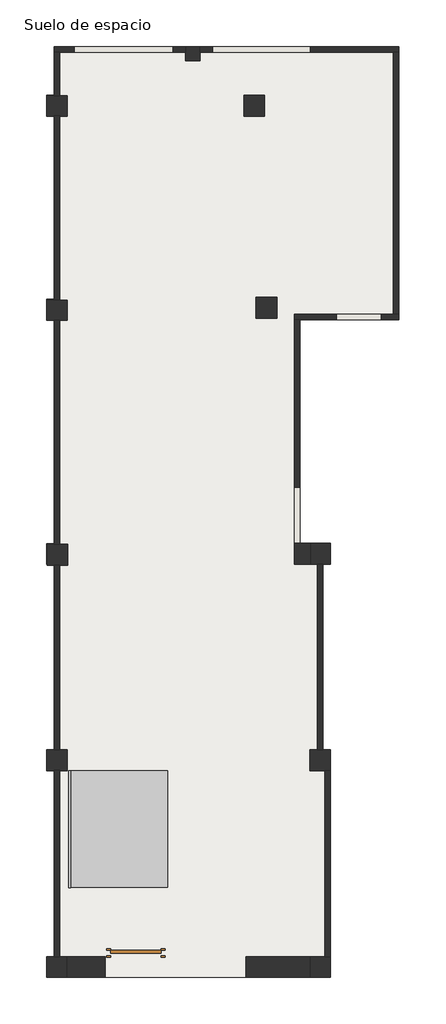
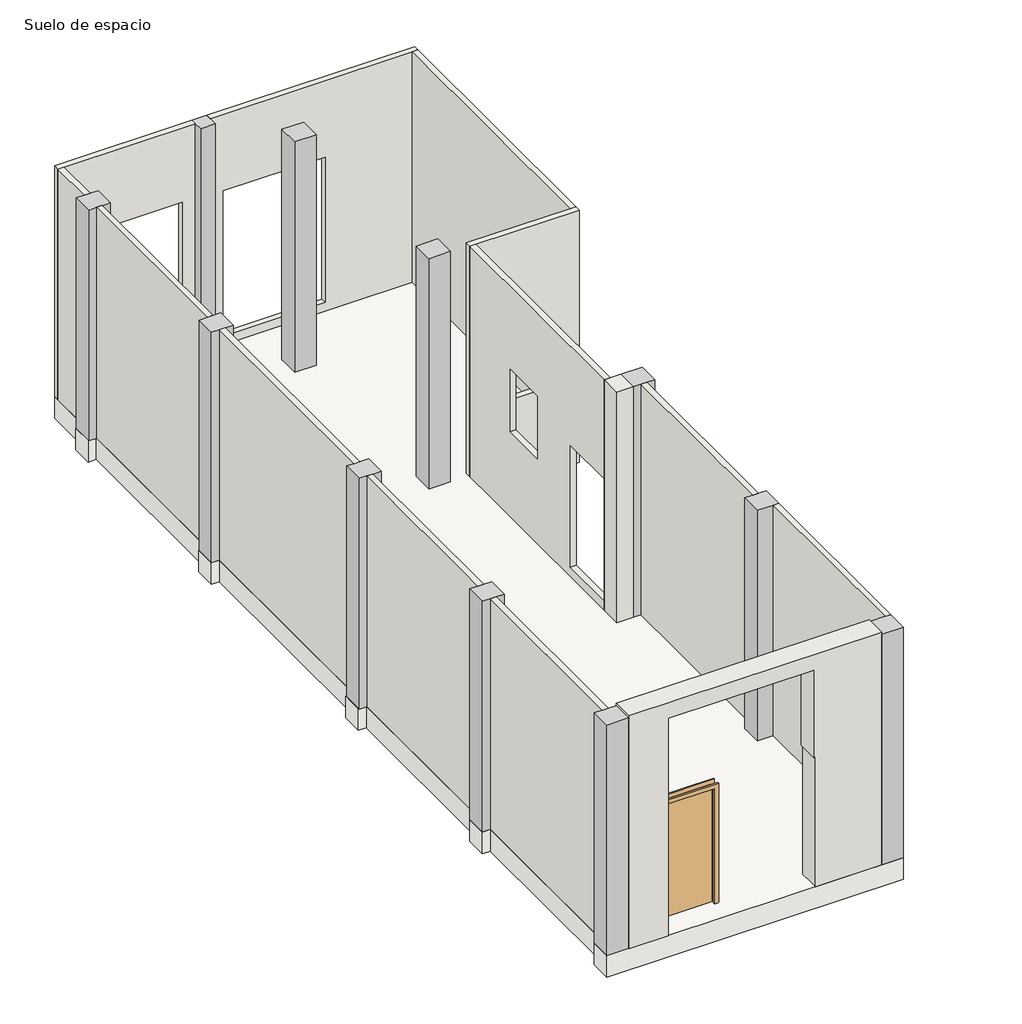
# One storey: 14 walls, 11 columns, 1 door, 1 railing, 1 ramp, 1 slab.
"""IFC4 building model written with IfcOpenShell, lengths in millimetres."""

import ifcopenshell
import ifcopenshell.guid

model = None  # the IFC model being written
_history = None  # IfcOwnerHistory: only IFC2X3 demands one
_inside = {}  # id of a spatial element -> (the spatial element, [elements in it])
_under = {}  # id of a project, library or spatial element -> (it, [spatial elements below it])
_declared = {}  # id of a project -> (the project, [libraries it declares])
_typed = {}  # id of a type object -> (the type object, [elements of that type])
_made_of = {}  # id of a material, layer set ... -> (it, [elements and type objects made of it])


def new_model(schema):
    """Start an empty IFC model of exactly this schema.

    Asked for "IFC4X3", IfcOpenShell would pick the latest addendum, in which some entities
    have other attributes; the version numbers below select the first issue.
    IFC2X3 requires an IfcOwnerHistory on every rooted entity: one is made here for all.
    """
    global model, _history
    if schema == "IFC4X3":
        model = ifcopenshell.file(schema_version=(4, 3, 0, 0))
    else:
        model = ifcopenshell.file(schema=schema)
    _inside.clear()
    _under.clear()
    _declared.clear()
    _typed.clear()
    _made_of.clear()
    _history = None
    if model.schema == "IFC2X3":
        org = make("IfcOrganization", Name="unknown")
        user = make(
            "IfcPersonAndOrganization",
            ThePerson=make("IfcPerson", FamilyName="unknown"),
            TheOrganization=org,
        )
        app = make(
            "IfcApplication",
            ApplicationDeveloper=org,
            Version="unknown",
            ApplicationFullName="unknown",
            ApplicationIdentifier="unknown",
        )
        _history = make(
            "IfcOwnerHistory",
            OwningUser=user,
            OwningApplication=app,
            ChangeAction="ADDED",
            CreationDate=0,
        )
    return model


def make(cls, **values):
    """One entity of the class cls with the attributes given. An attribute that is None is left unset."""
    return model.create_entity(
        cls, **{name: value for name, value in values.items() if value is not None}
    )


def rooted(cls, **values):
    """An entity with a GlobalId (a new one), such as an element, a storey or a relation."""
    return make(cls, GlobalId=ifcopenshell.guid.new(), OwnerHistory=_history, **values)


def si_unit(unit_type, name, prefix=None):
    """IfcSIUnit, for example si_unit("LENGTHUNIT", "METRE", prefix="MILLI")."""
    return make("IfcSIUnit", UnitType=unit_type, Prefix=prefix, Name=name)


def assignment(units):
    """IfcUnitAssignment: the units of a project."""
    return None if units is None else make("IfcUnitAssignment", Units=units)


def point(xyz):
    """IfcCartesianPoint."""
    return None if xyz is None else make("IfcCartesianPoint", Coordinates=xyz)


def direction(xyz):
    """IfcDirection."""
    return None if xyz is None else make("IfcDirection", DirectionRatios=xyz)


def frame(location, z_axis=None, x_axis=None):
    """IfcAxis2Placement3D, a coordinate frame: its origin and axes. An axis left out is left unset."""
    return make(
        "IfcAxis2Placement3D",
        Location=point(location),
        Axis=direction(z_axis),
        RefDirection=direction(x_axis),
    )


def origin():
    """The frame at (0, 0, 0) with its axes left unset."""
    return frame((0.0, 0.0, 0.0))


def origin_with_axes():
    """The frame at (0, 0, 0) with the z axis (0, 0, 1) and the x axis (1, 0, 0) written out."""
    return frame((0.0, 0.0, 0.0), z_axis=(0.0, 0.0, 1.0), x_axis=(1.0, 0.0, 0.0))


def place(relative_to, where):
    """IfcLocalPlacement: puts the frame where relative to a parent placement (None: the world)."""
    return make(
        "IfcLocalPlacement", PlacementRelTo=relative_to, RelativePlacement=where
    )


def context(
    kind, dimensions, precision=None, world=None, true_north=None, identifier=None
):
    """IfcGeometricRepresentationContext, for example the 3D "Model" context."""
    return make(
        "IfcGeometricRepresentationContext",
        ContextIdentifier=identifier,
        ContextType=kind,
        CoordinateSpaceDimension=dimensions,
        Precision=precision,
        WorldCoordinateSystem=world,
        TrueNorth=true_north,
    )


def project(units=None, contexts=None):
    """IfcProject with its units and contexts."""
    return rooted(
        "IfcProject",
        Name="project",
        RepresentationContexts=contexts,
        UnitsInContext=assignment(units),
    )


def spatial(cls, under=None, at=None, **own):
    """A site, building, storey or space (cls), placed at a placement, below another one or the project."""
    s = rooted(cls, ObjectPlacement=at, **own)
    if under is not None:
        _under.setdefault(under.id(), (under, []))[1].append(s)
    return s


def polyline(points):
    """IfcPolyline through the points."""
    return make("IfcPolyline", Points=[point(p) for p in points])


def ellipse_curve(where, semi_axis1, semi_axis2):
    """IfcEllipse in the frame where."""
    return make(
        "IfcEllipse", Position=where, SemiAxis1=semi_axis1, SemiAxis2=semi_axis2
    )


def outline(outer, holes=None, kind="AREA"):
    """IfcArbitraryClosedProfileDef: a profile drawn as a closed curve; with holes, ...WithVoids."""
    if holes is None:
        return make("IfcArbitraryClosedProfileDef", ProfileType=kind, OuterCurve=outer)
    return make(
        "IfcArbitraryProfileDefWithVoids",
        ProfileType=kind,
        OuterCurve=outer,
        InnerCurves=holes,
    )


def extrude(swept, where, along, depth):
    """IfcExtrudedAreaSolid: the profile swept, set in the frame where, extruded along a direction by depth."""
    return make(
        "IfcExtrudedAreaSolid",
        SweptArea=swept,
        Position=where,
        ExtrudedDirection=direction(along),
        Depth=depth,
    )


def faces_of(points, faces, orient=None, outer=None):
    """IfcFace entities. A face is a list of loops; a loop is a list of indices into points, from 0.

    orient and outer hold one flag for each loop. By default every Orientation is true, the
    first loop of a face is its IfcFaceOuterBound and the others are IfcFaceBound.
    """
    made = []
    for i, loops in enumerate(faces):
        bounds = []
        for j, loop in enumerate(loops):
            is_outer = j == 0 if outer is None else outer[i][j]
            bounds.append(
                make(
                    "IfcFaceOuterBound" if is_outer else "IfcFaceBound",
                    Bound=make("IfcPolyLoop", Polygon=[points[k] for k in loop]),
                    Orientation=True if orient is None else orient[i][j],
                )
            )
        made.append(make("IfcFace", Bounds=bounds))
    return made


def faceted_brep(points, faces, orient=None, outer=None, voids=None):
    """IfcFacetedBrep: a solid bounded by flat faces; with voids (closed shells), ...WithVoids."""
    shared = [point(p) for p in points]
    hull = make("IfcClosedShell", CfsFaces=faces_of(shared, faces, orient, outer))
    if voids is None:
        return make("IfcFacetedBrep", Outer=hull)
    return make(
        "IfcFacetedBrepWithVoids",
        Outer=hull,
        Voids=[
            make(cls, CfsFaces=faces_of(shared, fs, o, b)) for cls, fs, o, b in voids
        ],
    )


def shape(context_of_items, identifier, shape_type, items):
    """IfcShapeRepresentation: the items that make up one representation, for example the "Body"."""
    return make(
        "IfcShapeRepresentation",
        ContextOfItems=context_of_items,
        RepresentationIdentifier=identifier,
        RepresentationType=shape_type,
        Items=items,
    )


def source(mapping_origin, context_of_items, identifier, shape_type, items):
    """IfcRepresentationMap: a shape defined once, which mapped items show again and again."""
    return make(
        "IfcRepresentationMap",
        MappingOrigin=mapping_origin,
        MappedRepresentation=shape(context_of_items, identifier, shape_type, items),
    )


def transform(
    local_origin,
    x_axis=None,
    y_axis=None,
    z_axis=None,
    scale=None,
    scale2=None,
    scale3=None,
    uniform=True,
):
    """IfcCartesianTransformationOperator3D, or its non-uniform kind. x_axis, y_axis, z_axis: its Axis1, 2, 3."""
    if uniform:
        return make(
            "IfcCartesianTransformationOperator3D",
            Axis1=direction(x_axis),
            Axis2=direction(y_axis),
            LocalOrigin=point(local_origin),
            Scale=scale,
            Axis3=direction(z_axis),
        )
    return make(
        "IfcCartesianTransformationOperator3DnonUniform",
        Axis1=direction(x_axis),
        Axis2=direction(y_axis),
        LocalOrigin=point(local_origin),
        Scale=scale,
        Axis3=direction(z_axis),
        Scale2=scale2,
        Scale3=scale3,
    )


def mapped(mapping_source, mapping_target):
    """IfcMappedItem: shows the shape of a source again, moved by a transform."""
    return make(
        "IfcMappedItem", MappingSource=mapping_source, MappingTarget=mapping_target
    )


def made_of(thing, what):
    """Note that an element or type object is made of a material, layer set ...; save() writes the relation."""
    if what is not None:
        _made_of.setdefault(what.id(), (what, []))[1].append(thing)
    return thing


def element(
    cls,
    number,
    at=None,
    inside=None,
    cuts=None,
    type_object=None,
    material=None,
    context=None,
    identifier="Body",
    shape_type=None,
    held_by="IfcProductDefinitionShape",
    body=None,
    shapes=None,
    **own,
):
    """One element of the class cls, such as IfcWall. Its Tag is "e" and its number.

    at: its placement. inside: the storey or other place that contains it. cuts: it is an
    opening in that element (IfcRelVoidsElement). A single representation is given by context,
    identifier, shape_type and body (its items); several are given by shapes. held_by: the class
    of the entity that holds the representations. save() writes the other relations.
    """
    e = rooted(cls, Tag="e%d" % number, ObjectPlacement=at, **own)
    if body is not None:
        shapes = [shape(context, identifier, shape_type, body)]
    if shapes is not None:
        e.Representation = make(held_by, Representations=shapes)
    if inside is not None:
        _inside.setdefault(inside.id(), (inside, []))[1].append(e)
    if cuts is not None:
        rooted(
            "IfcRelVoidsElement", RelatingBuildingElement=cuts, RelatedOpeningElement=e
        )
    if type_object is not None:
        _typed.setdefault(type_object.id(), (type_object, []))[1].append(e)
    return made_of(e, material)


def aggregate(whole, parts):
    """IfcRelAggregates: a whole, such as a stair, and the parts it consists of."""
    return rooted("IfcRelAggregates", RelatingObject=whole, RelatedObjects=parts)


def save(model, path):
    """Write the relations noted so far, then the file.

    IfcRelAggregates (storeys below a building ...), IfcRelContainedInSpatialStructure (elements
    in a storey), IfcRelDefinesByType, IfcRelAssociatesMaterial and IfcRelDeclares: one each for
    every whole, place, type object, material and project.
    """
    for whole, parts in _under.values():
        aggregate(whole, parts)
    for where, things in _inside.values():
        rooted(
            "IfcRelContainedInSpatialStructure",
            RelatedElements=things,
            RelatingStructure=where,
        )
    for kind, things in _typed.values():
        rooted("IfcRelDefinesByType", RelatedObjects=things, RelatingType=kind)
    for what, things in _made_of.values():
        rooted("IfcRelAssociatesMaterial", RelatedObjects=things, RelatingMaterial=what)
    for by, libraries in _declared.values():
        rooted("IfcRelDeclares", RelatingContext=by, RelatedDefinitions=libraries)
    model.write(path)


def plane_surface(at):
    """IfcPlane: the flat surface through the origin of the frame at, square to its z axis."""
    return make("IfcPlane", Position=at)


def cylinder_surface(at, radius):
    """IfcCylindricalSurface: all points at the distance radius from the z axis of the frame at."""
    return make("IfcCylindricalSurface", Position=at, Radius=radius)


def advanced_brep(points, edges, surfaces, faces):
    """IfcAdvancedBrep: a solid bounded by faces that lie on surfaces and meet in shared edges.

    An edge is (start, end): straight between two places in points (the first is 0);
    or (start, end, curve); or (start, end, curve, False) where it runs against its curve.
    A face is (place in surfaces, loops), or (place, loops, False) where it looks against
    its surface's normal. A loop lists edges by number (the first is 1), with a minus sign
    where the edge is run from its end to its start. The first loop is the outer one.
    """
    corners = [point(p) for p in points]
    vertices = [make("IfcVertexPoint", VertexGeometry=c) for c in corners]
    made = []
    for start, end, *more in edges:
        made.append(
            make(
                "IfcEdgeCurve",
                EdgeStart=vertices[start],
                EdgeEnd=vertices[end],
                EdgeGeometry=more[0] if more else make("IfcPolyline", Points=[corners[start], corners[end]]),
                SameSense=more[1] if len(more) > 1 else True,
            )
        )
    hull = []
    for where, loops, *sense in faces:
        bounds = []
        for j, loop in enumerate(loops):
            ring = [make("IfcOrientedEdge", EdgeElement=made[abs(k) - 1], Orientation=k > 0) for k in loop]
            bounds.append(
                make(
                    "IfcFaceOuterBound" if j == 0 else "IfcFaceBound",
                    Bound=make("IfcEdgeLoop", EdgeList=ring),
                    Orientation=True,
                )
            )
        hull.append(make("IfcAdvancedFace", Bounds=bounds, FaceSurface=surfaces[where], SameSense=sense[0] if sense else True))
    return make("IfcAdvancedBrep", Outer=make("IfcClosedShell", CfsFaces=hull))


def m_rectangular_column_380_x_380mm_f7aa0fc7(model_context):
    return source(origin(), model_context, "Body", "SweptSolid", [
        extrude(outline(polyline([(190.0, 190.0), (190.0, -190.0), (-190.0, -190.0), (-190.0, 190.0), (190.0, 190.0)])), frame((0.0, 0.0, 40.0), z_axis=(0.0, 0.0, 1.0), x_axis=(1.0, 0.0, 0.0)), (0.0, 0.0, 1.0), 4260.0),
    ])


def m_single_flush_0915_x_2134mm_17617764(model_context):
    return source(origin(), model_context, "Body", "SweptSolid", [
        extrude(outline(polyline([(2210.0, -533.5), (0.0, -533.5), (0.0, -457.5), (2134.0, -457.5), (2134.0, 457.5), (0.0, 457.5), (0.0, 533.5), (2210.0, 533.5), (2210.0, -533.5)])), frame((0.0, -75.0, 0.0), z_axis=(0.0, 1.0, 0.0), x_axis=(0.0, 0.0, 1.0)), (0.0, 0.0, 1.0), 25.0),
        extrude(outline(polyline([(2210.0, 533.5), (2210.0, -533.5), (0.0, -533.5), (0.0, -457.5), (2134.0, -457.5), (2134.0, 457.5), (0.0, 457.5), (0.0, 533.5), (2210.0, 533.5)])), frame((0.0, 50.0, 0.0), z_axis=(0.0, 1.0, 0.0), x_axis=(0.0, 0.0, 1.0)), (0.0, 0.0, 1.0), 25.0),
        extrude(outline(polyline([(457.5, 1.0), (457.5, -50.0), (-457.5, -50.0), (-457.5, 1.0), (457.5, 1.0)])), origin_with_axes(), (0.0, 0.0, 1.0), 2134.0),
    ])


def ramp_1_445c0b72(model_context):
    return source(origin(), model_context, "Body", "SweptSolid", [
        extrude(outline(polyline([(-378.9025016, 40.0), (1760.7723822, 200.0), (1760.7723822, 49.5812066), (-378.9025016, -110.4187934), (-378.9025016, 40.0)])), frame((5764.7203549, 0.0, 0.0), z_axis=(1.0, 0.0, 0.0), x_axis=(0.0, 1.0, 0.0)), (0.0, 0.0, 1.0), 1790.0),
    ])


model = new_model("IFC4")

# Units and contexts
model_context = context("Model", 3, world=origin())
ifc_project = project(units=[si_unit("LENGTHUNIT", "METRE", prefix="MILLI")], contexts=[model_context])

# Site, building, storey
site = spatial("IfcSite", under=ifc_project)
building = spatial("IfcBuilding", under=site)
storey = spatial("IfcBuildingStorey", under=building, Name="Suelo de espacio", Elevation=40.0)

# Columns
placement = place(None, origin())
element("IfcColumn", 1, ObjectType="M_Rectangular Column : 260 x 260mm", at=placement, inside=storey, context=model_context, shape_type="Brep", body=[
    faceted_brep([(8142.3508412, 14950.939444, 4300.0), (7882.3508412, 14950.939444, 4300.0), (7882.3508412, 14850.939444, 4300.0), (7882.3508412, 14690.939444, 4300.0), (8142.3508412, 14690.939444, 4300.0), (8142.3508412, 14850.939444, 4300.0), (8142.3508412, 14950.939444, 40.0), (8142.3508412, 14850.939444, 40.0), (8142.3508412, 14690.939444, 40.0), (7882.3508412, 14690.939444, 40.0), (7882.3508412, 14850.939444, 40.0), (7882.3508412, 14950.939444, 40.0)], [[[0, 1, 2, 3, 4, 5]], [[6, 7, 8, 9, 10, 11]], [[1, 0, 6, 11]], [[3, 2, 1, 11, 10, 9]], [[4, 3, 9, 8]], [[0, 5, 4, 8, 7, 6]]]),
])
element("IfcColumn", 2, ObjectType="M_Rectangular Column : 380 x 370mm", at=placement, inside=storey, context=model_context, shape_type="Brep", body=[
    faceted_brep([(5722.3508412, 10330.939444, 4300.0), (5342.3508412, 10330.939444, 4300.0), (5342.3508412, 9960.939444, 4300.0), (5482.3508412, 9960.939444, 4300.0), (5582.3508412, 9960.939444, 4300.0), (5722.3508412, 9960.939444, 4300.0), (5722.3508412, 10330.939444, 40.0), (5722.3508412, 9960.939444, 40.0), (5582.3508412, 9960.939444, 40.0), (5482.3508412, 9960.939444, 40.0), (5342.3508412, 9960.939444, 40.0), (5342.3508412, 10330.939444, 40.0)], [[[0, 1, 2, 3, 4, 5]], [[6, 7, 8, 9, 10, 11]], [[1, 0, 6, 11]], [[2, 1, 11, 10]], [[5, 4, 3, 2, 10, 9, 8, 7]], [[0, 5, 7, 6]]]),
])
element("IfcColumn", 3, ObjectType="M_Rectangular Column : 380 x 370mm", at=placement, inside=storey, context=model_context, shape_type="Brep", body=[
    faceted_brep([(5722.3508412, 14050.939444, 4300.0), (5582.3508412, 14050.939444, 4300.0), (5482.3508412, 14050.939444, 4300.0), (5342.3508412, 14050.939444, 4300.0), (5342.3508412, 13680.939444, 4300.0), (5482.3508412, 13680.939444, 4300.0), (5482.3508412, 13685.939444, 4300.0), (5582.3508412, 13685.939444, 4300.0), (5582.3508412, 13680.939444, 4300.0), (5722.3508412, 13680.939444, 4300.0), (5722.3508412, 14050.939444, 40.0), (5722.3508412, 13680.939444, 40.0), (5582.3508412, 13680.939444, 40.0), (5582.3508412, 13685.939444, 40.0), (5482.3508412, 13685.939444, 40.0), (5482.3508412, 13680.939444, 40.0), (5342.3508412, 13680.939444, 40.0), (5342.3508412, 14050.939444, 40.0), (5482.3508412, 14050.939444, 40.0), (5582.3508412, 14050.939444, 40.0)], [[[0, 1, 2, 3, 4, 5, 6, 7, 8, 9]], [[10, 11, 12, 13, 14, 15, 16, 17, 18, 19]], [[3, 2, 1, 0, 10, 19, 18, 17]], [[4, 3, 17, 16]], [[4, 16, 15, 5]], [[0, 9, 11, 10]], [[7, 13, 12, 8]], [[14, 6, 5, 15]], [[13, 7, 6, 14]], [[11, 9, 8, 12]]]),
])
element("IfcColumn", 4, ObjectType="M_Rectangular Column : 380 x 380mm", at=placement, inside=storey, context=model_context, shape_type="Brep", body=[
    faceted_brep([(5722.3508412, -1629.060556, 4300.0), (5582.3508412, -1629.060556, 4300.0), (5482.3508412, -1629.060556, 4300.0), (5342.3508412, -1629.060556, 4300.0), (5342.3508412, -2009.060556, 4300.0), (5722.3508412, -2009.060556, 4300.0), (5722.3508412, -1629.060556, 40.0), (5722.3508412, -2009.060556, 40.0), (5342.3508412, -2009.060556, 40.0), (5342.3508412, -1629.060556, 40.0), (5482.3508412, -1629.060556, 40.0), (5582.3508412, -1629.060556, 40.0)], [[[0, 1, 2, 3, 4, 5]], [[6, 7, 8, 9, 10, 11]], [[3, 2, 1, 0, 6, 11, 10, 9]], [[4, 3, 9, 8]], [[5, 4, 8, 7]], [[0, 5, 7, 6]]]),
])
element("IfcColumn", 5, ObjectType="M_Rectangular Column : 380 x 380mm", at=placement, inside=storey, context=model_context, shape_type="Brep", body=[
    faceted_brep([(10522.3508412, -1629.060556, 4300.0), (10422.3508412, -1629.060556, 4300.0), (10142.3508412, -1629.060556, 4300.0), (10142.3508412, -2009.060556, 4300.0), (10522.3508412, -2009.060556, 4300.0), (10522.3508412, -1629.060556, 40.0), (10522.3508412, -2009.060556, 40.0), (10142.3508412, -2009.060556, 40.0), (10142.3508412, -1629.060556, 40.0), (10422.3508412, -1629.060556, 40.0)], [[[0, 1, 2, 3, 4]], [[5, 6, 7, 8, 9]], [[2, 1, 0, 5, 9, 8]], [[3, 2, 8, 7]], [[4, 3, 7, 6]], [[0, 4, 6, 5]]]),
])
element("IfcColumn", 6, ObjectType="M_Rectangular Column : 380 x 380mm", at=placement, inside=storey, context=model_context, shape_type="Brep", body=[
    faceted_brep([(5722.3508412, 2140.939444, 4300.0), (5582.3508412, 2140.939444, 4300.0), (5482.3508412, 2140.939444, 4300.0), (5342.3508412, 2140.939444, 4300.0), (5342.3508412, 1760.939444, 4300.0), (5482.3508412, 1760.939444, 4300.0), (5482.3508412, 1761.3849652, 4300.0), (5582.3508412, 1761.3849652, 4300.0), (5582.3508412, 1760.939444, 4300.0), (5722.3508412, 1760.939444, 4300.0), (5722.3508412, 2140.939444, 40.0), (5722.3508412, 1760.939444, 40.0), (5582.3508412, 1760.939444, 40.0), (5582.3508412, 1761.3849652, 40.0), (5482.3508412, 1761.3849652, 40.0), (5482.3508412, 1760.939444, 40.0), (5342.3508412, 1760.939444, 40.0), (5342.3508412, 2140.939444, 40.0), (5482.3508412, 2140.939444, 40.0), (5582.3508412, 2140.939444, 40.0)], [[[0, 1, 2, 3, 4, 5, 6, 7, 8, 9]], [[10, 11, 12, 13, 14, 15, 16, 17, 18, 19]], [[3, 2, 1, 0, 10, 19, 18, 17]], [[4, 3, 17, 16]], [[4, 16, 15, 5]], [[0, 9, 11, 10]], [[7, 13, 12, 8]], [[14, 6, 5, 15]], [[11, 9, 8, 12]], [[13, 7, 6, 14]]]),
])
element("IfcColumn", 7, ObjectType="M_Rectangular Column : 380 x 380mm", at=placement, inside=storey, context=model_context, shape_type="Brep", body=[
    faceted_brep([(10522.3508412, 2140.939444, 4300.0), (10382.3508412, 2140.939444, 4300.0), (10282.3508412, 2140.939444, 4300.0), (10142.3508412, 2140.939444, 4300.0), (10142.3508412, 1760.939444, 4300.0), (10422.3508412, 1760.939444, 4300.0), (10522.3508412, 1760.939444, 4300.0), (10522.3508412, 2140.939444, 40.0), (10522.3508412, 1760.939444, 40.0), (10422.3508412, 1760.939444, 40.0), (10142.3508412, 1760.939444, 40.0), (10142.3508412, 2140.939444, 40.0), (10282.3508412, 2140.939444, 40.0), (10382.3508412, 2140.939444, 40.0)], [[[0, 1, 2, 3, 4, 5, 6]], [[7, 8, 9, 10, 11, 12, 13]], [[3, 2, 1, 0, 7, 13, 12, 11]], [[4, 3, 11, 10]], [[6, 5, 4, 10, 9, 8]], [[0, 6, 8, 7]]]),
])
element("IfcColumn", 8, ObjectType="M_Rectangular Column : 380 x 380mm", at=placement, inside=storey, context=model_context, shape_type="Brep", body=[
    faceted_brep([(5732.3508412, 5880.939444, 4300.0), (5582.3508412, 5880.939444, 4300.0), (5482.3508412, 5880.939444, 4300.0), (5352.3508412, 5880.939444, 4300.0), (5352.3508412, 5500.939444, 4300.0), (5482.3508412, 5500.939444, 4300.0), (5582.3508412, 5500.939444, 4300.0), (5732.3508412, 5500.939444, 4300.0), (5732.3508412, 5880.939444, 40.0), (5732.3508412, 5500.939444, 40.0), (5582.3508412, 5500.939444, 40.0), (5482.3508412, 5500.939444, 40.0), (5352.3508412, 5500.939444, 40.0), (5352.3508412, 5880.939444, 40.0), (5482.3508412, 5880.939444, 40.0), (5582.3508412, 5880.939444, 40.0)], [[[0, 1, 2, 3, 4, 5, 6, 7]], [[8, 9, 10, 11, 12, 13, 14, 15]], [[3, 2, 1, 0, 8, 15, 14, 13]], [[4, 3, 13, 12]], [[7, 6, 5, 4, 12, 11, 10, 9]], [[0, 7, 9, 8]]]),
])
element("IfcColumn", 9, ObjectType="M_Rectangular Column : 380 x 380mm", at=placement, inside=storey, context=model_context, shape_type="Brep", body=[
    faceted_brep([(10522.3508412, 5520.939444, 4300.0), (10522.3508412, 5900.939444, 4300.0), (10152.3508412, 5900.939444, 4300.0), (10152.3508412, 5520.939444, 4300.0), (10282.3508412, 5520.939444, 4300.0), (10382.3508412, 5520.939444, 4300.0), (10522.3508412, 5900.939444, 40.0), (10522.3508412, 5520.939444, 40.0), (10382.3508412, 5520.939444, 40.0), (10282.3508412, 5520.939444, 40.0), (10152.3508412, 5520.939444, 40.0), (10152.3508412, 5900.939444, 40.0)], [[[0, 1, 2, 3, 4, 5]], [[6, 7, 8, 9, 10, 11]], [[1, 6, 11, 2]], [[7, 0, 5, 4, 3, 10, 9, 8]], [[1, 0, 7, 6]], [[3, 2, 11, 10]]]),
])
m_rectangular_column_380_x_380mm_shape = m_rectangular_column_380_x_380mm_f7aa0fc7(model_context)
element("IfcColumn", 10, ObjectType="M_Rectangular Column : 380 x 380mm", at=placement, inside=storey, context=model_context, shape_type="MappedRepresentation", body=[
    mapped(m_rectangular_column_380_x_380mm_shape, transform((9132.3508412, 13870.939444, 0.0), x_axis=(1.0, 0.0, 0.0), y_axis=(0.0, 1.0, 0.0), z_axis=(0.0, 0.0, 1.0))),
])
element("IfcColumn", 11, ObjectType="M_Rectangular Column : 380 x 380mm", at=placement, inside=storey, context=model_context, shape_type="MappedRepresentation", body=[
    mapped(m_rectangular_column_380_x_380mm_shape, transform((9352.3508412, 10190.939444, 0.0), x_axis=(1.0, 0.0, 0.0), y_axis=(0.0, 1.0, 0.0), z_axis=(0.0, 0.0, 1.0))),
])

# Door
m_single_flush_0915_x_2134mm_shape = m_single_flush_0915_x_2134mm_17617764(model_context)
element("IfcDoor", 12, ObjectType="M_Single-Flush : 0915 x 2134mm", at=placement, inside=storey, context=model_context, shape_type="MappedRepresentation", body=[
    mapped(m_single_flush_0915_x_2134mm_shape, transform((6972.3508412, -1564.060556, 40.0), x_axis=(-1.0, 0.0, 0.0), y_axis=(0.0, -1.0, 0.0), z_axis=(0.0, 0.0, 1.0))),
])

# Railing
element("IfcRailing", 13, ObjectType="900mm Pipe", at=placement, inside=storey, context=model_context, shape_type="AdvancedBrep", body=[
    advanced_brep(
    [(5784.7203549, -378.9025016, 919.9441609), (5744.7203549, -378.9025016, 919.9441609), (5784.7203549, 1760.7723822, 1079.9441609), (5744.7203549, 1760.7723822, 1079.9441609)],
    [
        (0, 1, ellipse_curve(frame((5764.7203549, -378.9025016, 919.9441609), z_axis=(0.0, -1.0, 0.0), x_axis=(0.0, 0.0, -1.0)), 20.0558391, 20.0)),
        (1, 0, ellipse_curve(frame((5764.7203549, -378.9025016, 919.9441609), z_axis=(0.0, -1.0, 0.0), x_axis=(0.0, 0.0, -1.0)), 20.0558391, 20.0)),
        (2, 3, ellipse_curve(frame((5764.7203549, 1760.7723822, 1079.9441609), z_axis=(0.0, 1.0, 0.0), x_axis=(0.0, 0.0, -1.0)), 20.0558391, 20.0)),
        (3, 2, ellipse_curve(frame((5764.7203549, 1760.7723822, 1079.9441609), z_axis=(0.0, 1.0, 0.0), x_axis=(0.0, 0.0, -1.0)), 20.0558391, 20.0)),
        (0, 2),
        (3, 1),
    ],
    [
        plane_surface(frame((5764.7203549, -378.9025016, 940.0), z_axis=(0.0, -1.0, 0.0), x_axis=(0.0, 0.0, 1.0))),
        plane_surface(frame((5764.7203549, 1760.7723822, 1100.0), z_axis=(0.0, 1.0, 0.0), x_axis=(0.0, 0.0, 1.0))),
        cylinder_surface(frame((5764.7203549, -377.4111112, 920.0556837), z_axis=(0.0, -0.9972158174462339, -0.07456952081809044), x_axis=(-1.0, 0.0, 0.0)), 20.0),
    ],
    [
        (0, [[1, 2]]),
        (1, [[3, 4]]),
        (2, [[-1, 5, -4, 6]]),
        (2, [[-2, -6, -3, -5]]),
    ],
),
    advanced_brep(
    [(5749.7203549, -378.9025016, 799.9581207), (5779.7203549, -378.9025016, 799.9581207), (5749.7203549, 1760.7723822, 959.9581207), (5779.7203549, 1760.7723822, 959.9581207)],
    [
        (0, 1, ellipse_curve(frame((5764.7203549, -378.9025016, 799.9581207), z_axis=(0.0, -1.0, 0.0), x_axis=(0.0, 0.0, -1.0)), 15.0418793, 15.0)),
        (1, 0, ellipse_curve(frame((5764.7203549, -378.9025016, 799.9581207), z_axis=(0.0, -1.0, 0.0), x_axis=(0.0, 0.0, -1.0)), 15.0418793, 15.0)),
        (2, 3, ellipse_curve(frame((5764.7203549, 1760.7723822, 959.9581207), z_axis=(0.0, 1.0, 0.0), x_axis=(0.0, 0.0, -1.0)), 15.0418793, 15.0)),
        (3, 2, ellipse_curve(frame((5764.7203549, 1760.7723822, 959.9581207), z_axis=(0.0, 1.0, 0.0), x_axis=(0.0, 0.0, -1.0)), 15.0418793, 15.0)),
        (0, 2),
        (3, 1),
    ],
    [
        plane_surface(frame((5764.7203549, -378.9025016, 815.0), z_axis=(0.0, -1.0, 0.0), x_axis=(0.0, 0.0, 1.0))),
        plane_surface(frame((5764.7203549, 1760.7723822, 975.0), z_axis=(0.0, 1.0, 0.0), x_axis=(0.0, 0.0, 1.0))),
        cylinder_surface(frame((5764.7203549, -377.7839588, 800.0417627), z_axis=(0.0, -0.9972158174462339, -0.07456952081809044), x_axis=(1.0, 0.0, 0.0)), 15.0),
    ],
    [
        (0, [[1, 2]]),
        (1, [[3, 4]]),
        (2, [[-1, 5, -4, 6]]),
        (2, [[-2, -6, -3, -5]]),
    ],
),
    advanced_brep(
    [(5749.7203549, -378.9025016, 674.9581207), (5779.7203549, -378.9025016, 674.9581207), (5749.7203549, 1760.7723822, 834.9581207), (5779.7203549, 1760.7723822, 834.9581207)],
    [
        (0, 1, ellipse_curve(frame((5764.7203549, -378.9025016, 674.9581207), z_axis=(0.0, -1.0, 0.0), x_axis=(0.0, 0.0, -1.0)), 15.0418793, 15.0)),
        (1, 0, ellipse_curve(frame((5764.7203549, -378.9025016, 674.9581207), z_axis=(0.0, -1.0, 0.0), x_axis=(0.0, 0.0, -1.0)), 15.0418793, 15.0)),
        (2, 3, ellipse_curve(frame((5764.7203549, 1760.7723822, 834.9581207), z_axis=(0.0, 1.0, 0.0), x_axis=(0.0, 0.0, -1.0)), 15.0418793, 15.0)),
        (3, 2, ellipse_curve(frame((5764.7203549, 1760.7723822, 834.9581207), z_axis=(0.0, 1.0, 0.0), x_axis=(0.0, 0.0, -1.0)), 15.0418793, 15.0)),
        (0, 2),
        (3, 1),
    ],
    [
        plane_surface(frame((5764.7203549, -378.9025016, 690.0), z_axis=(0.0, -1.0, 0.0), x_axis=(0.0, 0.0, 1.0))),
        plane_surface(frame((5764.7203549, 1760.7723822, 850.0), z_axis=(0.0, 1.0, 0.0), x_axis=(0.0, 0.0, 1.0))),
        cylinder_surface(frame((5764.7203549, -377.7839588, 675.0417627), z_axis=(0.0, -0.9972158174462339, -0.07456952081809044), x_axis=(1.0, 0.0, 0.0)), 15.0),
    ],
    [
        (0, [[1, 2]]),
        (1, [[3, 4]]),
        (2, [[-1, 5, -4, 6]]),
        (2, [[-2, -6, -3, -5]]),
    ],
),
    advanced_brep(
    [(5749.7203549, -378.9025016, 549.9581207), (5779.7203549, -378.9025016, 549.9581207), (5749.7203549, 1760.7723822, 709.9581207), (5779.7203549, 1760.7723822, 709.9581207)],
    [
        (0, 1, ellipse_curve(frame((5764.7203549, -378.9025016, 549.9581207), z_axis=(0.0, -1.0, 0.0), x_axis=(0.0, 0.0, -1.0)), 15.0418793, 15.0)),
        (1, 0, ellipse_curve(frame((5764.7203549, -378.9025016, 549.9581207), z_axis=(0.0, -1.0, 0.0), x_axis=(0.0, 0.0, -1.0)), 15.0418793, 15.0)),
        (2, 3, ellipse_curve(frame((5764.7203549, 1760.7723822, 709.9581207), z_axis=(0.0, 1.0, 0.0), x_axis=(0.0, 0.0, -1.0)), 15.0418793, 15.0)),
        (3, 2, ellipse_curve(frame((5764.7203549, 1760.7723822, 709.9581207), z_axis=(0.0, 1.0, 0.0), x_axis=(0.0, 0.0, -1.0)), 15.0418793, 15.0)),
        (0, 2),
        (3, 1),
    ],
    [
        plane_surface(frame((5764.7203549, -378.9025016, 565.0), z_axis=(0.0, -1.0, 0.0), x_axis=(0.0, 0.0, 1.0))),
        plane_surface(frame((5764.7203549, 1760.7723822, 725.0), z_axis=(0.0, 1.0, 0.0), x_axis=(0.0, 0.0, 1.0))),
        cylinder_surface(frame((5764.7203549, -377.7839588, 550.0417627), z_axis=(0.0, -0.9972158174462339, -0.07456952081809044), x_axis=(1.0, 0.0, 0.0)), 15.0),
    ],
    [
        (0, [[1, 2]]),
        (1, [[3, 4]]),
        (2, [[-1, 5, -4, 6]]),
        (2, [[-2, -6, -3, -5]]),
    ],
),
    advanced_brep(
    [(5749.7203549, -378.9025016, 424.9581207), (5779.7203549, -378.9025016, 424.9581207), (5749.7203549, 1760.7723822, 584.9581207), (5779.7203549, 1760.7723822, 584.9581207)],
    [
        (0, 1, ellipse_curve(frame((5764.7203549, -378.9025016, 424.9581207), z_axis=(0.0, -1.0, 0.0), x_axis=(0.0, 0.0, -1.0)), 15.0418793, 15.0)),
        (1, 0, ellipse_curve(frame((5764.7203549, -378.9025016, 424.9581207), z_axis=(0.0, -1.0, 0.0), x_axis=(0.0, 0.0, -1.0)), 15.0418793, 15.0)),
        (2, 3, ellipse_curve(frame((5764.7203549, 1760.7723822, 584.9581207), z_axis=(0.0, 1.0, 0.0), x_axis=(0.0, 0.0, -1.0)), 15.0418793, 15.0)),
        (3, 2, ellipse_curve(frame((5764.7203549, 1760.7723822, 584.9581207), z_axis=(0.0, 1.0, 0.0), x_axis=(0.0, 0.0, -1.0)), 15.0418793, 15.0)),
        (0, 2),
        (3, 1),
    ],
    [
        plane_surface(frame((5764.7203549, -378.9025016, 440.0), z_axis=(0.0, -1.0, 0.0), x_axis=(0.0, 0.0, 1.0))),
        plane_surface(frame((5764.7203549, 1760.7723822, 600.0), z_axis=(0.0, 1.0, 0.0), x_axis=(0.0, 0.0, 1.0))),
        cylinder_surface(frame((5764.7203549, -377.7839588, 425.0417627), z_axis=(0.0, -0.9972158174462339, -0.07456952081809044), x_axis=(1.0, 0.0, 0.0)), 15.0),
    ],
    [
        (0, [[1, 2]]),
        (1, [[3, 4]]),
        (2, [[-1, 5, -4, 6]]),
        (2, [[-2, -6, -3, -5]]),
    ],
),
    advanced_brep(
    [(5749.7203549, -378.9025016, 299.9581207), (5779.7203549, -378.9025016, 299.9581207), (5749.7203549, 1760.7723822, 459.9581207), (5779.7203549, 1760.7723822, 459.9581207)],
    [
        (0, 1, ellipse_curve(frame((5764.7203549, -378.9025016, 299.9581207), z_axis=(0.0, -1.0, 0.0), x_axis=(0.0, 0.0, -1.0)), 15.0418793, 15.0)),
        (1, 0, ellipse_curve(frame((5764.7203549, -378.9025016, 299.9581207), z_axis=(0.0, -1.0, 0.0), x_axis=(0.0, 0.0, -1.0)), 15.0418793, 15.0)),
        (2, 3, ellipse_curve(frame((5764.7203549, 1760.7723822, 459.9581207), z_axis=(0.0, 1.0, 0.0), x_axis=(0.0, 0.0, -1.0)), 15.0418793, 15.0)),
        (3, 2, ellipse_curve(frame((5764.7203549, 1760.7723822, 459.9581207), z_axis=(0.0, 1.0, 0.0), x_axis=(0.0, 0.0, -1.0)), 15.0418793, 15.0)),
        (0, 2),
        (3, 1),
    ],
    [
        plane_surface(frame((5764.7203549, -378.9025016, 315.0), z_axis=(0.0, -1.0, 0.0), x_axis=(0.0, 0.0, 1.0))),
        plane_surface(frame((5764.7203549, 1760.7723822, 475.0), z_axis=(0.0, 1.0, 0.0), x_axis=(0.0, 0.0, 1.0))),
        cylinder_surface(frame((5764.7203549, -377.7839588, 300.0417627), z_axis=(0.0, -0.9972158174462339, -0.07456952081809044), x_axis=(1.0, 0.0, 0.0)), 15.0),
    ],
    [
        (0, [[1, 2]]),
        (1, [[3, 4]]),
        (2, [[-1, 5, -4, 6]]),
        (2, [[-2, -6, -3, -5]]),
    ],
),
    advanced_brep(
    [(5749.7203549, -378.9025016, 174.9581207), (5779.7203549, -378.9025016, 174.9581207), (5749.7203549, 1760.7723822, 334.9581207), (5779.7203549, 1760.7723822, 334.9581207)],
    [
        (0, 1, ellipse_curve(frame((5764.7203549, -378.9025016, 174.9581207), z_axis=(0.0, -1.0, 0.0), x_axis=(0.0, 0.0, -0.9999999999999999)), 15.0418793, 15.0)),
        (1, 0, ellipse_curve(frame((5764.7203549, -378.9025016, 174.9581207), z_axis=(0.0, -1.0, 0.0), x_axis=(0.0, 0.0, -0.9999999999999999)), 15.0418793, 15.0)),
        (2, 3, ellipse_curve(frame((5764.7203549, 1760.7723822, 334.9581207), z_axis=(0.0, 1.0, 0.0), x_axis=(0.0, 0.0, -0.9999999999999999)), 15.0418793, 15.0)),
        (3, 2, ellipse_curve(frame((5764.7203549, 1760.7723822, 334.9581207), z_axis=(0.0, 1.0, 0.0), x_axis=(0.0, 0.0, -0.9999999999999999)), 15.0418793, 15.0)),
        (0, 2),
        (3, 1),
    ],
    [
        plane_surface(frame((5764.7203549, -378.9025016, 190.0), z_axis=(0.0, -1.0, 0.0), x_axis=(0.0, 0.0, 1.0))),
        plane_surface(frame((5764.7203549, 1760.7723822, 350.0), z_axis=(0.0, 1.0, 0.0), x_axis=(0.0, 0.0, 1.0))),
        cylinder_surface(frame((5764.7203549, -377.7839588, 175.0417627), z_axis=(0.0, -0.9972158174462339, -0.07456952081809042), x_axis=(1.0, 0.0, 0.0)), 15.0),
    ],
    [
        (0, [[1, 2]]),
        (1, [[3, 4]]),
        (2, [[-1, 5, -4, 6]]),
        (2, [[-2, -6, -3, -5]]),
    ],
),
    advanced_brep(
    [(5777.2203549, 1621.0974984, 1049.443753), (5777.2203549, 1621.0974984, 189.5554313), (5752.2203549, 1621.0974984, 189.5554313), (5752.2203549, 1621.0974984, 1049.443753)],
    [
        (0, 1),
        (1, 2, ellipse_curve(frame((5764.7203549, 1621.0974984, 189.5554313), z_axis=(0.0, -0.07456952081809026, 0.9972158174462339), x_axis=(0.0, 0.9972158174462339, 0.07456952081808967)), 12.5348994, 12.5)),
        (2, 3),
        (3, 0, ellipse_curve(frame((5764.7203549, 1621.0974984, 1049.443753), z_axis=(0.0, 0.07456952081809023, -0.9972158174462339), x_axis=(0.0, 0.9972158174462339, 0.0745695208180897)), 12.5348994, 12.5)),
        (0, 3, ellipse_curve(frame((5764.7203549, 1621.0974984, 1049.443753), z_axis=(0.0, 0.07456952081809023, -0.9972158174462339), x_axis=(0.0, 0.9972158174462339, 0.0745695208180897)), 12.5348994, 12.5)),
        (2, 1, ellipse_curve(frame((5764.7203549, 1621.0974984, 189.5554313), z_axis=(0.0, -0.07456952081809026, 0.9972158174462339), x_axis=(0.0, 0.9972158174462339, 0.07456952081808967)), 12.5348994, 12.5)),
    ],
    [
        cylinder_surface(frame((5764.7203549, 1621.0974984, 89.5554313), z_axis=(0.0, 0.0, 1.0), x_axis=(-1.0, 0.0, 0.0)), 12.5),
        plane_surface(frame((5739.7203549, 1646.0974984, 1051.3131959), z_axis=(0.0, -0.07456952081809023, 0.9972158174462339), x_axis=(1.0, 0.0, 0.0))),
        plane_surface(frame((5739.7203549, 1596.0974984, 187.6859884), z_axis=(0.0, 0.07456952081809026, -0.9972158174462339), x_axis=(1.0, 0.0, 0.0))),
    ],
    [
        (0, [[1, 2, 3, 4]]),
        (0, [[-1, 5, -3, 6]]),
        (1, [[-4, -5]]),
        (2, [[-2, -6]]),
    ],
),
    advanced_brep(
    [(5777.2203549, 621.0974984, 974.6660374), (5777.2203549, 621.0974984, 114.7777156), (5752.2203549, 621.0974984, 114.7777156), (5752.2203549, 621.0974984, 974.6660374)],
    [
        (0, 1),
        (1, 2, ellipse_curve(frame((5764.7203549, 621.0974984, 114.7777156), z_axis=(0.0, -0.07456952081809026, 0.9972158174462339), x_axis=(0.0, 0.9972158174462339, 0.07456952081808967)), 12.5348994, 12.5)),
        (2, 3),
        (3, 0, ellipse_curve(frame((5764.7203549, 621.0974984, 974.6660374), z_axis=(0.0, 0.07456952081809023, -0.9972158174462339), x_axis=(0.0, 0.9972158174462339, 0.0745695208180897)), 12.5348994, 12.5)),
        (0, 3, ellipse_curve(frame((5764.7203549, 621.0974984, 974.6660374), z_axis=(0.0, 0.07456952081809023, -0.9972158174462339), x_axis=(0.0, 0.9972158174462339, 0.0745695208180897)), 12.5348994, 12.5)),
        (2, 1, ellipse_curve(frame((5764.7203549, 621.0974984, 114.7777156), z_axis=(0.0, -0.07456952081809026, 0.9972158174462339), x_axis=(0.0, 0.9972158174462339, 0.07456952081808967)), 12.5348994, 12.5)),
    ],
    [
        cylinder_surface(frame((5764.7203549, 621.0974984, 14.7777156), z_axis=(0.0, 0.0, 1.0), x_axis=(-1.0, 0.0, 0.0)), 12.5),
        plane_surface(frame((5739.7203549, 646.0974984, 976.5354803), z_axis=(0.0, -0.07456952081809023, 0.9972158174462339), x_axis=(1.0, 0.0, 0.0))),
        plane_surface(frame((5739.7203549, 596.0974984, 112.9082727), z_axis=(0.0, 0.07456952081809026, -0.9972158174462339), x_axis=(1.0, 0.0, 0.0))),
    ],
    [
        (0, [[1, 2, 3, 4]]),
        (0, [[-1, 5, -3, 6]]),
        (1, [[-4, -5]]),
        (2, [[-2, -6]]),
    ],
),
    advanced_brep(
    [(5777.2203549, 1748.2723822, 1058.9536003), (5777.2203549, 1748.2723822, 199.0652786), (5752.2203549, 1748.2723822, 199.0652786), (5752.2203549, 1748.2723822, 1058.9536003)],
    [
        (0, 1),
        (1, 2, ellipse_curve(frame((5764.7203549, 1748.2723822, 199.0652786), z_axis=(0.0, -0.07456952081809026, 0.9972158174462339), x_axis=(0.0, 0.9972158174462339, 0.07456952081808967)), 12.5348994, 12.5)),
        (2, 3),
        (3, 0, ellipse_curve(frame((5764.7203549, 1748.2723822, 1058.9536003), z_axis=(0.0, 0.07456952081809023, -0.9972158174462339), x_axis=(0.0, 0.9972158174462339, 0.0745695208180897)), 12.5348994, 12.5)),
        (0, 3, ellipse_curve(frame((5764.7203549, 1748.2723822, 1058.9536003), z_axis=(0.0, 0.07456952081809023, -0.9972158174462339), x_axis=(0.0, 0.9972158174462339, 0.0745695208180897)), 12.5348994, 12.5)),
        (2, 1, ellipse_curve(frame((5764.7203549, 1748.2723822, 199.0652786), z_axis=(0.0, -0.07456952081809026, 0.9972158174462339), x_axis=(0.0, 0.9972158174462339, 0.07456952081808967)), 12.5348994, 12.5)),
    ],
    [
        cylinder_surface(frame((5764.7203549, 1748.2723822, 99.0652786), z_axis=(0.0, 0.0, 1.0), x_axis=(-1.0, 0.0, 0.0)), 12.5),
        plane_surface(frame((5739.7203549, 1773.2723822, 1060.8230432), z_axis=(0.0, -0.07456952081809023, 0.9972158174462339), x_axis=(1.0, 0.0, 0.0))),
        plane_surface(frame((5739.7203549, 1723.2723822, 197.1958357), z_axis=(0.0, 0.07456952081809026, -0.9972158174462339), x_axis=(1.0, 0.0, 0.0))),
    ],
    [
        (0, [[1, 2, 3, 4]]),
        (0, [[-1, 5, -3, 6]]),
        (1, [[-4, -5]]),
        (2, [[-2, -6]]),
    ],
),
    advanced_brep(
    [(5777.2203549, -366.4025016, 900.8230432), (5777.2203549, -366.4025016, 40.9347214), (5752.2203549, -366.4025016, 40.9347214), (5752.2203549, -366.4025016, 900.8230432)],
    [
        (0, 1),
        (1, 2, ellipse_curve(frame((5764.7203549, -366.4025016, 40.9347214), z_axis=(0.0, -0.07456952081809026, 0.9972158174462339), x_axis=(0.0, 0.9972158174462339, 0.07456952081808967)), 12.5348994, 12.5)),
        (2, 3),
        (3, 0, ellipse_curve(frame((5764.7203549, -366.4025016, 900.8230432), z_axis=(0.0, 0.07456952081809023, -0.9972158174462339), x_axis=(0.0, 0.9972158174462339, 0.0745695208180897)), 12.5348994, 12.5)),
        (0, 3, ellipse_curve(frame((5764.7203549, -366.4025016, 900.8230432), z_axis=(0.0, 0.07456952081809023, -0.9972158174462339), x_axis=(0.0, 0.9972158174462339, 0.0745695208180897)), 12.5348994, 12.5)),
        (2, 1, ellipse_curve(frame((5764.7203549, -366.4025016, 40.9347214), z_axis=(0.0, -0.07456952081809026, 0.9972158174462339), x_axis=(0.0, 0.9972158174462339, 0.07456952081808967)), 12.5348994, 12.5)),
    ],
    [
        cylinder_surface(frame((5764.7203549, -366.4025016, -59.0652786), z_axis=(0.0, 0.0, 1.0), x_axis=(-1.0, 0.0, 0.0)), 12.5),
        plane_surface(frame((5739.7203549, -341.4025016, 902.6924861), z_axis=(0.0, -0.07456952081809023, 0.9972158174462339), x_axis=(1.0, 0.0, 0.0))),
        plane_surface(frame((5739.7203549, -391.4025016, 39.0652786), z_axis=(0.0, 0.07456952081809026, -0.9972158174462339), x_axis=(1.0, 0.0, 0.0))),
    ],
    [
        (0, [[1, 2, 3, 4]]),
        (0, [[-1, 5, -3, 6]]),
        (1, [[-4, -5]]),
        (2, [[-2, -6]]),
    ],
),
])

# Ramp
ramp_1_shape = ramp_1_445c0b72(model_context)
element("IfcRamp", 14, ObjectType="Ramp 1", at=placement, inside=storey, context=model_context, shape_type="MappedRepresentation", body=[
    mapped(ramp_1_shape, transform((0.0, 0.0, 0.0), x_axis=(1.0, 0.0, 0.0), y_axis=(0.0, 1.0, 0.0), z_axis=(0.0, 0.0, 1.0))),
])

# Slab
element("IfcSlab", 15, ObjectType="Generic Floor - 400mm", at=placement, inside=storey, context=model_context, shape_type="SweptSolid", body=[
    extrude(outline(polyline([(11772.3508412, 14950.939444), (11772.3508412, 9970.939444), (9962.3508412, 9970.939444), (9962.3508412, 5900.939444), (10382.3508412, 5900.939444), (10382.3508412, 2140.939444), (10522.3508412, 2140.939444), (10522.3508412, -2009.060556), (5342.3508412, -2009.060556), (5342.3508412, -1629.060556), (5482.3508412, -1629.060556), (5482.3508412, 1761.3849652), (5342.3508412, 1761.3849652), (5342.3508412, 2140.939444), (5482.3508412, 2140.939444), (5482.3508412, 5516.6200626), (5342.3508412, 5516.6200626), (5342.3508412, 5896.6200626), (5482.3508412, 5896.6200626), (5482.3508412, 9965.939444), (5342.3508412, 9965.939444), (5342.3508412, 10345.939444), (5482.3508412, 10345.939444), (5482.3508412, 13690.939444), (5342.3508412, 13690.939444), (5342.3508412, 14060.939444), (5482.3508412, 14060.939444), (5482.3508412, 14950.939444), (11772.3508412, 14950.939444)])), frame((0.0, 0.0, -360.0), z_axis=(0.0, 0.0, 1.0), x_axis=(1.0, 0.0, 0.0)), (0.0, 0.0, 1.0), 400.0),
])

# Walls
element("IfcWall", 16, ObjectType="Generic - 100mm Masonry", at=placement, inside=storey, context=model_context, shape_type="Brep", body=[
    faceted_brep([(5582.3508412, -1629.060556, 40.0), (5582.3508412, 1760.939444, 40.0), (5582.3508412, 1761.3849652, 40.0), (5582.3508412, 1761.3849652, 4300.0), (5582.3508412, 1760.939444, 4300.0), (5582.3508412, -1629.060556, 4300.0), (5482.3508412, -1629.060556, 40.0), (5482.3508412, -1629.060556, 4300.0), (5482.3508412, 1760.939444, 4300.0), (5482.3508412, 1761.3849652, 4300.0), (5482.3508412, 1761.3849652, 40.0), (5482.3508412, 1760.939444, 40.0)], [[[0, 1, 2, 3, 4, 5]], [[6, 7, 8, 9, 10, 11]], [[2, 1, 0, 6, 11, 10]], [[3, 2, 10, 9]], [[5, 4, 3, 9, 8, 7]], [[0, 5, 7, 6]]]),
])
element("IfcWall", 17, ObjectType="Generic - 100mm Masonry", at=placement, inside=storey, context=model_context, shape_type="SweptSolid", body=[
    extrude(outline(polyline([(5582.3508412, 5500.939444), (5582.3508412, 2140.939444), (5482.3508412, 2140.939444), (5482.3508412, 5500.939444), (5582.3508412, 5500.939444)])), frame((0.0, 0.0, 40.0), z_axis=(0.0, 0.0, 1.0), x_axis=(1.0, 0.0, 0.0)), (0.0, 0.0, 1.0), 4260.0),
])
element("IfcWall", 18, ObjectType="Generic - 100mm Masonry", at=placement, inside=storey, context=model_context, shape_type="SweptSolid", body=[
    extrude(outline(polyline([(5582.3508412, 9960.939444), (5582.3508412, 5880.939444), (5482.3508412, 5880.939444), (5482.3508412, 9960.939444), (5582.3508412, 9960.939444)])), frame((0.0, 0.0, 40.0), z_axis=(0.0, 0.0, 1.0), x_axis=(1.0, 0.0, 0.0)), (0.0, 0.0, 1.0), 4260.0),
])
element("IfcWall", 19, ObjectType="Generic - 100mm Masonry", at=placement, inside=storey, context=model_context, shape_type="Brep", body=[
    faceted_brep([(5582.3508412, 10335.939444, 40.0), (5582.3508412, 13680.939444, 40.0), (5582.3508412, 13685.939444, 40.0), (5582.3508412, 13685.939444, 4300.0), (5582.3508412, 13680.939444, 4300.0), (5582.3508412, 10335.939444, 4300.0), (5482.3508412, 10335.939444, 40.0), (5482.3508412, 10335.939444, 4300.0), (5482.3508412, 13680.939444, 4300.0), (5482.3508412, 13685.939444, 4300.0), (5482.3508412, 13685.939444, 40.0), (5482.3508412, 13680.939444, 40.0)], [[[0, 1, 2, 3, 4, 5]], [[6, 7, 8, 9, 10, 11]], [[2, 1, 0, 6, 11, 10]], [[3, 2, 10, 9]], [[5, 4, 3, 9, 8, 7]], [[0, 5, 7, 6]]]),
])
element("IfcWall", 20, ObjectType="Generic - 100mm Masonry", at=placement, inside=storey, context=model_context, shape_type="SweptSolid", body=[
    extrude(outline(polyline([(5582.3508412, 14850.939444), (5582.3508412, 14050.939444), (5482.3508412, 14050.939444), (5482.3508412, 14850.939444), (5582.3508412, 14850.939444)])), frame((0.0, 0.0, 40.0), z_axis=(0.0, 0.0, 1.0), x_axis=(1.0, 0.0, 0.0)), (0.0, 0.0, 1.0), 4260.0),
])
element("IfcWall", 21, ObjectType="Generic - 100mm Masonry", at=placement, inside=storey, context=model_context, shape_type="Brep", body=[
    faceted_brep([(5482.3508412, 14850.939444, 40.0), (5582.3508412, 14850.939444, 40.0), (7882.3508412, 14850.939444, 40.0), (7882.3508412, 14850.939444, 4300.0), (5582.3508412, 14850.939444, 4300.0), (5482.3508412, 14850.939444, 4300.0), (5847.3508412, 14850.939444, 2924.0), (7651.3508412, 14850.939444, 2924.0), (7651.3508412, 14850.939444, 200.0), (5847.3508412, 14850.939444, 200.0), (7882.3508412, 14950.939444, 40.0), (5482.3508412, 14950.939444, 40.0), (5482.3508412, 14950.939444, 4300.0), (7882.3508412, 14950.939444, 4300.0), (7651.3508412, 14950.939444, 2924.0), (5847.3508412, 14950.939444, 2924.0), (5847.3508412, 14950.939444, 200.0), (7651.3508412, 14950.939444, 200.0)], [[[0, 1, 2, 3, 4, 5], [6, 7, 8, 9]], [[10, 11, 12, 13], [14, 15, 16, 17]], [[2, 1, 0, 11, 10]], [[3, 2, 10, 13]], [[5, 4, 3, 13, 12]], [[0, 5, 12, 11]], [[6, 15, 14, 7]], [[8, 17, 16, 9]], [[15, 6, 9, 16]], [[7, 14, 17, 8]]]),
])
element("IfcWall", 22, ObjectType="Generic - 100mm Masonry", at=placement, inside=storey, context=model_context, shape_type="Brep", body=[
    faceted_brep([(8142.3508412, 14850.939444, 40.0), (11672.3508412, 14850.939444, 40.0), (11772.3508412, 14850.939444, 40.0), (11772.3508412, 14850.939444, 4300.0), (11672.3508412, 14850.939444, 4300.0), (8142.3508412, 14850.939444, 4300.0), (8368.3508412, 14850.939444, 2885.0), (10154.3508412, 14850.939444, 2885.0), (10154.3508412, 14850.939444, 200.0), (8368.3508412, 14850.939444, 200.0), (11772.3508412, 14950.939444, 40.0), (8142.3508412, 14950.939444, 40.0), (8142.3508412, 14950.939444, 4300.0), (11772.3508412, 14950.939444, 4300.0), (10154.3508412, 14950.939444, 2885.0), (8368.3508412, 14950.939444, 2885.0), (8368.3508412, 14950.939444, 200.0), (10154.3508412, 14950.939444, 200.0)], [[[0, 1, 2, 3, 4, 5], [6, 7, 8, 9]], [[10, 11, 12, 13], [14, 15, 16, 17]], [[2, 1, 0, 11, 10]], [[5, 4, 3, 13, 12]], [[0, 5, 12, 11]], [[3, 2, 10, 13]], [[6, 15, 14, 7]], [[8, 17, 16, 9]], [[15, 6, 9, 16]], [[7, 14, 17, 8]]]),
])
element("IfcWall", 23, ObjectType="Generic - 100mm Masonry", at=placement, inside=storey, context=model_context, shape_type="SweptSolid", body=[
    extrude(outline(polyline([(11672.3508412, 10070.939444), (11672.3508412, 14850.939444), (11772.3508412, 14850.939444), (11772.3508412, 10070.939444), (11672.3508412, 10070.939444)])), frame((0.0, 0.0, 40.0), z_axis=(0.0, 0.0, 1.0), x_axis=(1.0, 0.0, 0.0)), (0.0, 0.0, 1.0), 4260.0),
])
element("IfcWall", 24, ObjectType="Generic - 100mm Masonry", at=placement, inside=storey, context=model_context, shape_type="Brep", body=[
    faceted_brep([(11772.3508412, 10070.939444, 40.0), (11672.3508412, 10070.939444, 40.0), (9862.3508412, 10070.939444, 40.0), (9862.3508412, 10070.939444, 4300.0), (11672.3508412, 10070.939444, 4300.0), (11772.3508412, 10070.939444, 4300.0), (11452.3508412, 10070.939444, 2225.0), (10632.3508412, 10070.939444, 2225.0), (10632.3508412, 10070.939444, 1215.0), (11452.3508412, 10070.939444, 1215.0), (9862.3508412, 9970.939444, 40.0), (9962.3508412, 9970.939444, 40.0), (11772.3508412, 9970.939444, 40.0), (11772.3508412, 9970.939444, 4300.0), (9962.3508412, 9970.939444, 4300.0), (9862.3508412, 9970.939444, 4300.0), (10632.3508412, 9970.939444, 2225.0), (11452.3508412, 9970.939444, 2225.0), (11452.3508412, 9970.939444, 1215.0), (10632.3508412, 9970.939444, 1215.0)], [[[0, 1, 2, 3, 4, 5], [6, 7, 8, 9]], [[10, 11, 12, 13, 14, 15], [16, 17, 18, 19]], [[2, 1, 0, 12, 11, 10]], [[5, 4, 3, 15, 14, 13]], [[3, 2, 10, 15]], [[0, 5, 13, 12]], [[6, 17, 16, 7]], [[8, 19, 18, 9]], [[17, 6, 9, 18]], [[7, 16, 19, 8]]]),
])
element("IfcWall", 25, ObjectType="Generic - 100mm Masonry", at=placement, inside=storey, context=model_context, shape_type="SweptSolid", body=[
    extrude(outline(polyline([(9970.939444, 40.0), (5900.939444, 40.0), (5900.939444, 4300.0), (9970.939444, 4300.0), (9970.939444, 40.0)]), holes=[polyline([(8748.939444, 2766.0), (7928.939444, 2766.0), (7928.939444, 1616.0), (8748.939444, 1616.0), (8748.939444, 2766.0)]), polyline([(6925.939444, 2460.0), (5905.939444, 2460.0), (5905.939444, 220.0), (6925.939444, 220.0), (6925.939444, 2460.0)])]), frame((9862.3508412, 0.0, 0.0), z_axis=(1.0, 0.0, 0.0), x_axis=(0.0, 1.0, 0.0)), (0.0, 0.0, 1.0), 100.0),
])
element("IfcWall", 26, ObjectType="Generic - 100mm Masonry", at=placement, inside=storey, context=model_context, shape_type="SweptSolid", body=[
    extrude(outline(polyline([(10282.3508412, 2140.939444), (10282.3508412, 5520.939444), (10382.3508412, 5520.939444), (10382.3508412, 2140.939444), (10282.3508412, 2140.939444)])), frame((0.0, 0.0, 40.0), z_axis=(0.0, 0.0, 1.0), x_axis=(1.0, 0.0, 0.0)), (0.0, 0.0, 1.0), 4260.0),
])
element("IfcWall", 27, ObjectType="Generic - 100mm Masonry", at=placement, inside=storey, context=model_context, shape_type="SweptSolid", body=[
    extrude(outline(polyline([(10422.3508412, -1629.060556), (10422.3508412, 1760.939444), (10522.3508412, 1760.939444), (10522.3508412, -1629.060556), (10422.3508412, -1629.060556)])), frame((0.0, 0.0, 40.0), z_axis=(0.0, 0.0, 1.0), x_axis=(1.0, 0.0, 0.0)), (0.0, 0.0, 1.0), 4260.0),
])
element("IfcWall", 28, ObjectType="Generic - 380mm Masonry", at=placement, inside=storey, context=model_context, shape_type="Brep", body=[
    faceted_brep([(9862.3508412, 5520.939444, 40.0), (10152.3508412, 5520.939444, 40.0), (10152.3508412, 5520.939444, 4300.0), (9862.3508412, 5520.939444, 4300.0), (9862.3508412, 5900.939444, 40.0), (9862.3508412, 5900.939444, 4300.0), (9962.3508412, 5900.939444, 4300.0), (10152.3508412, 5900.939444, 4300.0), (10152.3508412, 5900.939444, 40.0), (9962.3508412, 5900.939444, 40.0)], [[[0, 1, 2, 3]], [[4, 5, 6, 7, 8, 9]], [[1, 0, 4, 9, 8]], [[2, 1, 8, 7]], [[3, 2, 7, 6, 5]], [[0, 3, 5, 4]]]),
])
element("IfcWall", 29, ObjectType="Generic - 380mm Masonry", at=placement, inside=storey, context=model_context, shape_type="Brep", body=[
    faceted_brep([(10142.3508412, -2009.060556, 40.0), (10142.3508412, -2009.060556, 4300.0), (10142.3508412, -2009.060556, 4340.0), (5722.3508412, -2009.060556, 4340.0), (5722.3508412, -2009.060556, 4300.0), (5722.3508412, -2009.060556, 40.0), (6412.3508412, -2009.060556, 40.0), (6412.3508412, -2009.060556, 3080.0), (6412.3508412, -2009.060556, 4050.0), (8952.3508412, -2009.060556, 4050.0), (8952.3508412, -2009.060556, 3080.0), (8952.3508412, -2009.060556, 2438.4), (8983.3912604, -2009.060556, 2438.4), (8983.3912604, -2009.060556, 40.0), (10142.3508412, -1629.060556, 4340.0), (10142.3508412, -1629.060556, 4300.0), (10142.3508412, -1629.060556, 40.0), (8983.3912604, -1629.060556, 40.0), (8983.3912604, -1629.060556, 2438.4), (8952.3508412, -1629.060556, 2438.4), (8952.3508412, -1629.060556, 4050.0), (6412.3508412, -1629.060556, 4050.0), (6412.3508412, -1629.060556, 40.0), (5722.3508412, -1629.060556, 40.0), (5722.3508412, -1629.060556, 4300.0), (5722.3508412, -1629.060556, 4340.0), (6412.3508412, -1929.060556, 4050.0), (8952.3508412, -1929.060556, 4050.0)], [[[0, 1, 2, 3, 4, 5, 6, 7, 8, 9, 10, 11, 12, 13]], [[14, 15, 16, 17, 18, 19, 20, 21, 22, 23, 24, 25]], [[5, 23, 22, 6]], [[16, 0, 13, 17]], [[2, 1, 0, 16, 15, 14]], [[3, 2, 14, 25]], [[5, 4, 3, 25, 24, 23]], [[18, 12, 11, 19]], [[12, 18, 17, 13]], [[8, 26, 21, 20, 27, 9]], [[21, 26, 8, 7, 6, 22]], [[9, 27, 20, 19, 11, 10]]]),
])

save(model, "model.ifc")

# Revit data of these elements
# Project information
#   Organization Name = "SHV"
#   Building Name = "Pere Valencia"
#   Author = "Ian Salter"
#   Project Issue Date = "Issue Date"
#   Project Status = "Project  Status"
#   Client Name = "Ian Salter"
#   Project Address = "## Street\nCity, State  Zip"
#   Project Name = "Project Name"
#   Project Number = "Project  Number"
# Type "M_Rectangular Column : 260 x 260mm"
#   Depth = 26.0 cm
#   Offset Base = 0.0 cm
#   Offset Top = 0.0 cm
#   Width = 26.0 cm
#   Material = none
# Type "M_Rectangular Column : 380 x 370mm"
#   Depth = 37.0 cm
#   Offset Base = 0.0 cm
#   Offset Top = 0.0 cm
#   Width = 38.0 cm
#   Material = none
# Type "M_Rectangular Column : 380 x 380mm"
#   Depth = 38.0 cm
#   Offset Base = 0.0 cm
#   Offset Top = 0.0 cm
#   Width = 38.0 cm
#   Material = none
# Type "M_Single-Flush : 0915 x 2134mm"
#   Type Mark = "15"
#   Thickness = 5.1 cm
#   Height = 213.4 cm
#   Trim Projection Ext = 2.5 cm
#   Trim Projection Int = 2.5 cm
#   Trim Width = 7.6 cm
#   Width = 91.5 cm
#   Door Material = Door - Panel
#   Frame Material = Door - Frame
#   Function = (empty or 0)
#   Wall Closure = (empty or 0)
# Type "900mm Pipe"
#   built-in parameter 1008612 = 0.019685 (stored number, unit not read)
#   built-in parameter 1008611 = 0.0984252 (stored number, unit not read)
#   built-in parameter 1008609 = 6.56168 (stored number, unit not read)
#   built-in parameter 1008604 = 0.19685 (stored number, unit not read)
#   built-in parameter 1008603 = 0.164042 (stored number, unit not read)
#   Railing Height = 90.0 cm
#   built-in parameter 1008630 = 2
#   built-in parameter 1008610 = 2
#   built-in parameter 1008605 = 1
#   built-in parameter 1008618 = M_Baluster - Round : 25mm
# Type "Ramp 1"
#   built-in parameter 1008304 = 0.492126 (stored number, unit not read)
#   built-in parameter 1008303 = 39.3701 (stored number, unit not read)
#   built-in parameter 1008301 = 12 (stored number, unit not read)
#   Function = 0
# Type "Generic Floor - 400mm"
#   Function = 0
#   Layers, outside or top first: 40.0 cm no material (function 1)
# Type "Generic - 100mm Masonry"
#   Layers, outside or top first: 10.0 cm "Concrete, Cast-in-Place gray" (function 1)
# Type "Generic - 380mm Masonry"
#   Layers, outside or top first: 38.0 cm "Concrete, Cast-in-Place gray" (function 1)
# Element 1 (IfcColumn, "M_Rectangular Column : 260 x 260mm")
#   Phase Created = Existing
#   Materials on its faces: "Concrete, Cast-in-Place gray"
# Elements 2, 3 (IfcColumn, "M_Rectangular Column : 380 x 370mm")
#   Phase Created = Existing
#   Materials on its faces: "Concrete, Cast-in-Place gray"
# Elements 4, 5 (IfcColumn, "M_Rectangular Column : 380 x 380mm")
#   Phase Created = New Construction
#   Materials on its faces: "Concrete, Cast-in-Place gray"
# Elements 6, 7, 8, 9 (IfcColumn, "M_Rectangular Column : 380 x 380mm")
#   Phase Created = Existing
#   Materials on its faces: "Concrete, Cast-in-Place gray"
# Elements 10, 11 (IfcColumn, "M_Rectangular Column : 380 x 380mm")
#   Phase Created = Existing
# Element 12 (IfcDoor, "M_Single-Flush : 0915 x 2134mm")
#   Phase Created = New Construction
#   Materials on its faces: "Door - Frame", "Door - Panel"
# Element 13 (IfcRailing, "900mm Pipe")
#   Phase Created = New Construction
# Element 14 (IfcRamp, "Ramp 1")
#   built-in parameter 1007275 = "DN"
#   built-in parameter 1007272 = "UP"
#   Width = 179.0 cm
#   built-in parameter 1007276 = 1
#   built-in parameter 1007274 = 1
#   built-in parameter 1007273 = 1
#   built-in parameter 1007271 = 1
#   Phase Created = New Construction
